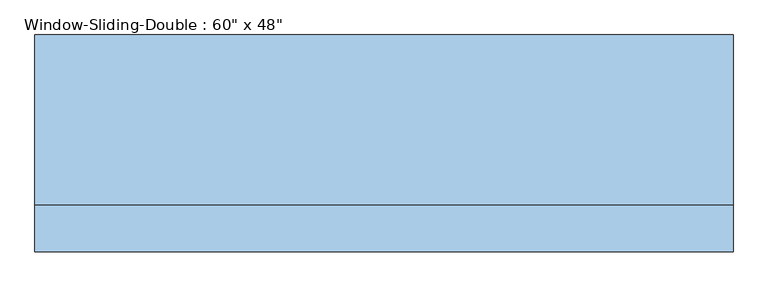
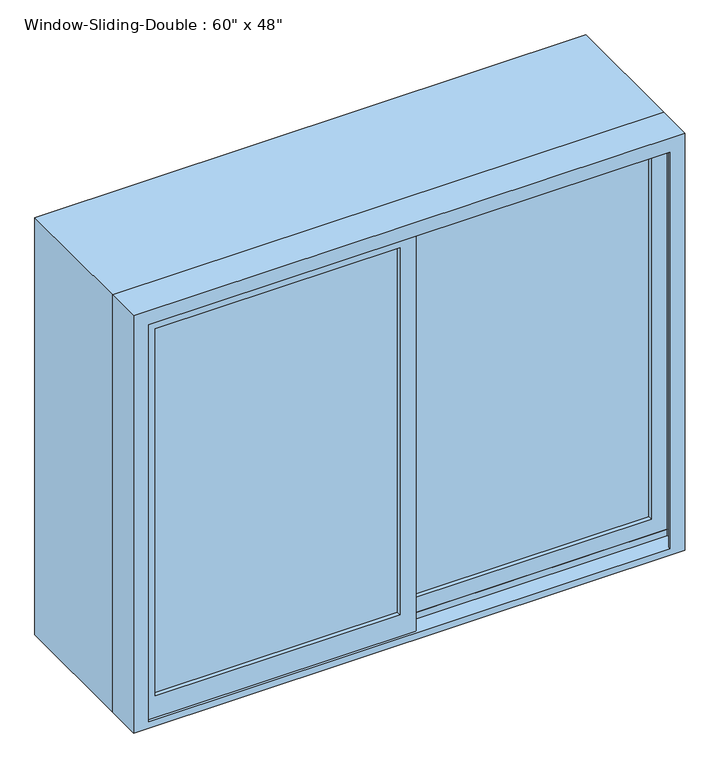
"""IFC4 building model written with IfcOpenShell, lengths in millimetres: window geometry."""

from ifc_helpers import new_model, si_unit, frame, origin, place, context, project, spatial, polyline, outline, extrude, faceted_brep, source, transform, mapped, element, save


def window_814bde12(model_context):
    return source(origin(), model_context, "Body", "SolidModel", [
        faceted_brep([(-762.0, -140.6525, 914.4), (762.0, -140.6525, 914.4), (762.0, -242.2525, 914.4), (-762.0, -242.2525, 914.4), (-721.0778905, -242.2525, 2092.6778905), (-721.0778905, -242.2525, 933.45), (-721.0778905, -235.9025, 933.45), (-721.0778905, -235.9025, 2092.6778905), (-742.95, -235.9025, 933.45), (-742.95, -235.9025, 2114.55), (742.95, -235.9025, 2114.55), (742.95, -235.9025, 933.45), (721.0778905, -235.9025, 933.45), (721.0778905, -235.9025, 2092.6778905), (-742.95, -191.4525, 933.45), (-742.95, -191.4525, 952.5), (-742.95, -147.0025, 952.5), (-742.95, -147.0025, 933.45), (-742.95, -140.6525, 933.45), (-742.95, -140.6525, 2114.55), (-762.0, -140.6525, 2133.6), (762.0, -140.6525, 2133.6), (742.95, -140.6525, 2114.55), (742.95, -140.6525, 933.45), (-762.0, -242.2525, 2133.6), (762.0, -242.2525, 2133.6), (721.0778905, -242.2525, 2092.6778905), (721.0778905, -242.2525, 933.45), (742.95, -147.0025, 933.45), (742.95, -147.0025, 952.5), (742.95, -191.4525, 952.5), (742.95, -191.4525, 933.45)], [[[0, 1, 2, 3]], [[4, 5, 6, 7]], [[7, 6, 8, 9, 10, 11, 12, 13]], [[9, 8, 14, 15, 16, 17, 18, 19]], [[0, 20, 21, 1], [22, 19, 18, 23]], [[24, 20, 0, 3]], [[2, 25, 24, 3], [4, 26, 27, 5]], [[7, 13, 26, 4]], [[9, 19, 22, 10]], [[20, 24, 25, 21]], [[13, 12, 27, 26]], [[22, 23, 28, 29, 30, 31, 11, 10]], [[21, 25, 2, 1]], [[27, 12, 11, 31, 14, 8, 6, 5]], [[31, 30, 15, 14]], [[30, 29, 16, 15]], [[29, 28, 17, 16]], [[18, 17, 28, 23]]]),
        extrude(outline(polyline([(2133.6, 762.0), (2133.6, -762.0), (914.4, -762.0), (914.4, 762.0), (2133.6, 762.0)]), holes=[polyline([(2114.55, -742.95), (2114.55, 742.95), (933.45, 742.95), (933.45, -742.95), (2114.55, -742.95)])]), frame((0.0, -140.6525, 0.0), z_axis=(0.0, 1.0, 0.0), x_axis=(0.0, 0.0, 1.0)), (0.0, 0.0, 1.0), 371.475),
        extrude(outline(polyline([(698.5, -178.7525), (22.225, -178.7525), (22.225, -172.4025), (698.5, -172.4025), (698.5, -178.7525)])), frame((0.0, 0.0, 996.95), z_axis=(0.0, 0.0, 1.0), x_axis=(1.0, 0.0, 0.0)), (0.0, 0.0, 1.0), 1073.15),
        extrude(outline(polyline([(698.5, -166.0525), (22.225, -166.0525), (22.225, -159.7025), (698.5, -159.7025), (698.5, -166.0525)])), frame((0.0, 0.0, 996.95), z_axis=(0.0, 0.0, 1.0), x_axis=(1.0, 0.0, 0.0)), (0.0, 0.0, 1.0), 1073.15),
        extrude(outline(polyline([(-22.225, -223.2025), (-698.5, -223.2025), (-698.5, -216.8525), (-22.225, -216.8525), (-22.225, -223.2025)])), frame((0.0, 0.0, 996.95), z_axis=(0.0, 0.0, 1.0), x_axis=(1.0, 0.0, 0.0)), (0.0, 0.0, 1.0), 1073.15),
        extrude(outline(polyline([(-22.225, -210.5025), (-698.5, -210.5025), (-698.5, -204.1525), (-22.225, -204.1525), (-22.225, -210.5025)])), frame((0.0, 0.0, 996.95), z_axis=(0.0, 0.0, 1.0), x_axis=(1.0, 0.0, 0.0)), (0.0, 0.0, 1.0), 1073.15),
        extrude(outline(polyline([(933.45, 22.225), (2114.55, 22.225), (2114.55, -742.95), (933.45, -742.95), (933.45, 22.225)]), holes=[polyline([(2070.1, -698.5), (2070.1, -22.225), (996.95, -22.225), (996.95, -698.5), (2070.1, -698.5)])]), frame((0.0, -235.9025, 0.0), z_axis=(0.0, 1.0, 0.0), x_axis=(0.0, 0.0, 1.0)), (0.0, 0.0, 1.0), 44.45),
        extrude(outline(polyline([(952.5, -22.225), (952.5, 742.95), (2114.55, 742.95), (2114.55, -22.225), (952.5, -22.225)]), holes=[polyline([(996.95, 698.5), (996.95, 22.225), (2070.1, 22.225), (2070.1, 698.5), (996.95, 698.5)])]), frame((0.0, -191.4525, 0.0), z_axis=(0.0, 1.0, 0.0), x_axis=(0.0, 0.0, 1.0)), (0.0, 0.0, 1.0), 44.45),
    ])


if __name__ == "__main__":
    model = new_model("IFC4")
    model_context = context("Model", 3, world=origin())
    ifc_project = project(units=[si_unit("LENGTHUNIT", "METRE", prefix="MILLI")], contexts=[model_context])
    site = spatial("IfcSite", under=ifc_project)
    building = spatial("IfcBuilding", under=site)
    placement = place(None, origin())
    window_shape = window_814bde12(model_context)
    element("IfcWindow", 1, ObjectType="Window-Sliding-Double : 60\" x 48\"", at=placement, inside=building, context=model_context, shape_type="MappedRepresentation", body=[
        mapped(window_shape, transform((0.0, 0.0, 0.0), x_axis=(1.0, 0.0, 0.0), y_axis=(0.0, 1.0, 0.0), z_axis=(0.0, 0.0, 1.0))),
    ])
    save(model, "model.ifc")

# Revit data of these elements
# Type "Window-Sliding-Double : 60\" x 48\""
#   Type Mark = "13"
#   Fire Rating = "0.5h"
#   Assembly Code = "B2020100"
#   Analytic Construction = "Double glazing - domestic"
#   Window Inset [instance default] = 0' - 0"
#   Wall Thickness [instance default] = 0' - 6"
#   Visual Light Transmittance = 0.81
#   Thermal Resistance (R) = 1.8146 (h·ft²·°F)/BTU
#   Solar Heat Gain Coefficient = 0.76
#   Muntin Width = 2' - 2 5/8"
#   Muntin Height = 3' - 6 1/4"
#   Interior Wall Closure [instance default] = 0' - 2 3/4"
#   Heat Transfer Coefficient (U) = 0.5511 BTU/(h·ft²·°F)
#   Frame Extension [instance default] = 0' - 0 1/4"
#   Exterior Wall Closure [instance default] = 0' - 1 1/4"
#   Rough Width = 5' - 0 1/2"
#   Rough Height = 4' - 0 1/2"
#   Height = 4' - 0"
#   Extension Jamb [instance default] = 0' - 2 3/4"
#   Default Sill Height = 3' - 0"
#   Width = 5' - 0"
#   Interior Trim Visibility [instance default] = yes
#   Indicator Visibility [instance default] = yes
#   Exterior Trim Visibility [instance default] = yes
#   Muntin Visibility = yes
#   Extension Jamb Visibility [instance default] = yes
#   Define Thermal Properties by = 1
#   Muntin Pattern = Muntin Pattern_2x2 : Muntin Pattern_2x2
#   Interior Trim Material = Cherry
#   Interior Trim = Trim-Window-Interior-Flat : Picture Frame
#   Interior Frame Material = Cherry
#   Glass Panel Material = Glass, Clear Glazing
#   Exterior Trim Material = PVC, Flexible
#   Exterior Trim = Trim-Window-Exterior-Flat : with Sill
#   Exterior Frame Material = PVC, Flexible
#   Wall Closure = (empty or 0)
# Element 1 (IfcWindow, "Window-Sliding-Double : 60\" x 48\"")
#   Wall Thickness = 1' - 5 7/8"
#   Extension Jamb = 1' - 2 5/8"
#   Materials on its faces: "Cherry", "Glass, Clear Glazing", "PVC, Flexible"
# Materials
#   "Cherry": class "Wood", colour RGB 157 77 38, transparency 0, Description = "Prunus Serotina", Cost = 0
#   "Glass, Clear Glazing": class "Glass", colour RGB 120 120 120, transparency 0, Description = "Clear glazing", Cost = 0
#   "PVC, Flexible": class "Plastic", colour RGB 178 178 178, transparency 0, Description = "Flexible polyvinyl chloride", Cost = 0
